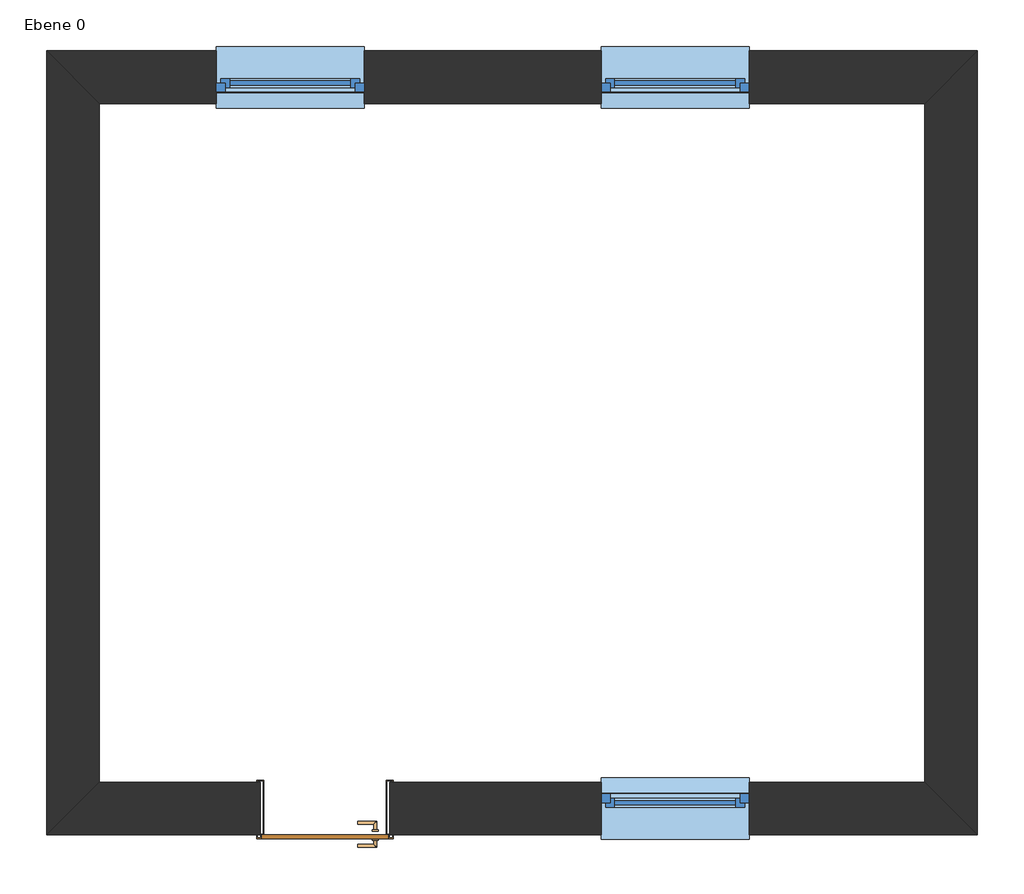
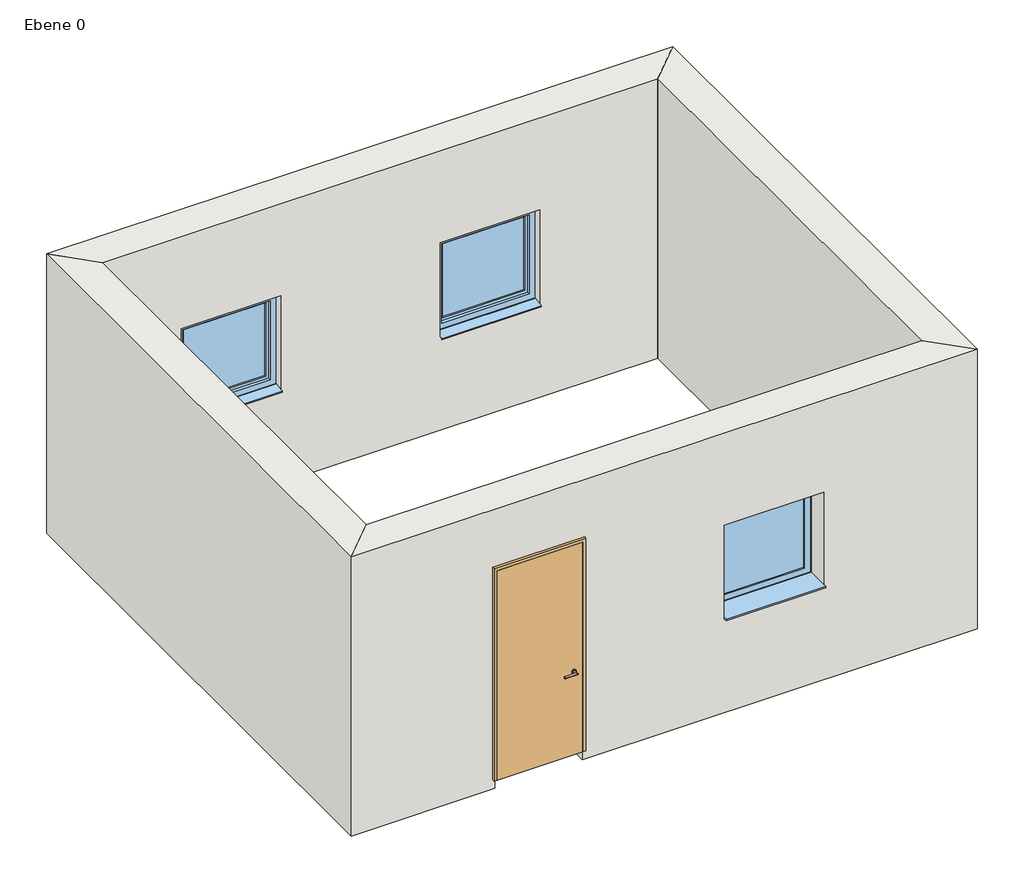
# One storey: 4 walls, 3 windows, 1 door.
"""IFC4 building model written with IfcOpenShell, lengths in millimetres."""

import ifcopenshell
import ifcopenshell.guid

model = None  # the IFC model being written
_history = None  # IfcOwnerHistory: only IFC2X3 demands one
_inside = {}  # id of a spatial element -> (the spatial element, [elements in it])
_under = {}  # id of a project, library or spatial element -> (it, [spatial elements below it])
_declared = {}  # id of a project -> (the project, [libraries it declares])
_typed = {}  # id of a type object -> (the type object, [elements of that type])
_made_of = {}  # id of a material, layer set ... -> (it, [elements and type objects made of it])


def new_model(schema):
    """Start an empty IFC model of exactly this schema.

    Asked for "IFC4X3", IfcOpenShell would pick the latest addendum, in which some entities
    have other attributes; the version numbers below select the first issue.
    IFC2X3 requires an IfcOwnerHistory on every rooted entity: one is made here for all.
    """
    global model, _history
    if schema == "IFC4X3":
        model = ifcopenshell.file(schema_version=(4, 3, 0, 0))
    else:
        model = ifcopenshell.file(schema=schema)
    _inside.clear()
    _under.clear()
    _declared.clear()
    _typed.clear()
    _made_of.clear()
    _history = None
    if model.schema == "IFC2X3":
        org = make("IfcOrganization", Name="unknown")
        user = make(
            "IfcPersonAndOrganization",
            ThePerson=make("IfcPerson", FamilyName="unknown"),
            TheOrganization=org,
        )
        app = make(
            "IfcApplication",
            ApplicationDeveloper=org,
            Version="unknown",
            ApplicationFullName="unknown",
            ApplicationIdentifier="unknown",
        )
        _history = make(
            "IfcOwnerHistory",
            OwningUser=user,
            OwningApplication=app,
            ChangeAction="ADDED",
            CreationDate=0,
        )
    return model


def make(cls, **values):
    """One entity of the class cls with the attributes given. An attribute that is None is left unset."""
    return model.create_entity(
        cls, **{name: value for name, value in values.items() if value is not None}
    )


def rooted(cls, **values):
    """An entity with a GlobalId (a new one), such as an element, a storey or a relation."""
    return make(cls, GlobalId=ifcopenshell.guid.new(), OwnerHistory=_history, **values)


def si_unit(unit_type, name, prefix=None):
    """IfcSIUnit, for example si_unit("LENGTHUNIT", "METRE", prefix="MILLI")."""
    return make("IfcSIUnit", UnitType=unit_type, Prefix=prefix, Name=name)


def assignment(units):
    """IfcUnitAssignment: the units of a project."""
    return None if units is None else make("IfcUnitAssignment", Units=units)


def point(xyz):
    """IfcCartesianPoint."""
    return None if xyz is None else make("IfcCartesianPoint", Coordinates=xyz)


def direction(xyz):
    """IfcDirection."""
    return None if xyz is None else make("IfcDirection", DirectionRatios=xyz)


def frame(location, z_axis=None, x_axis=None):
    """IfcAxis2Placement3D, a coordinate frame: its origin and axes. An axis left out is left unset."""
    return make(
        "IfcAxis2Placement3D",
        Location=point(location),
        Axis=direction(z_axis),
        RefDirection=direction(x_axis),
    )


def frame_2d(location, x_axis=None):
    """IfcAxis2Placement2D, a coordinate frame in the plane: its origin and x axis."""
    return make(
        "IfcAxis2Placement2D", Location=point(location), RefDirection=direction(x_axis)
    )


def origin():
    """The frame at (0, 0, 0) with its axes left unset."""
    return frame((0.0, 0.0, 0.0))


def origin_with_axes():
    """The frame at (0, 0, 0) with the z axis (0, 0, 1) and the x axis (1, 0, 0) written out."""
    return frame((0.0, 0.0, 0.0), z_axis=(0.0, 0.0, 1.0), x_axis=(1.0, 0.0, 0.0))


def place(relative_to, where):
    """IfcLocalPlacement: puts the frame where relative to a parent placement (None: the world)."""
    return make(
        "IfcLocalPlacement", PlacementRelTo=relative_to, RelativePlacement=where
    )


def context(
    kind, dimensions, precision=None, world=None, true_north=None, identifier=None
):
    """IfcGeometricRepresentationContext, for example the 3D "Model" context."""
    return make(
        "IfcGeometricRepresentationContext",
        ContextIdentifier=identifier,
        ContextType=kind,
        CoordinateSpaceDimension=dimensions,
        Precision=precision,
        WorldCoordinateSystem=world,
        TrueNorth=true_north,
    )


def project(units=None, contexts=None):
    """IfcProject with its units and contexts."""
    return rooted(
        "IfcProject",
        Name="project",
        RepresentationContexts=contexts,
        UnitsInContext=assignment(units),
    )


def spatial(cls, under=None, at=None, **own):
    """A site, building, storey or space (cls), placed at a placement, below another one or the project."""
    s = rooted(cls, ObjectPlacement=at, **own)
    if under is not None:
        _under.setdefault(under.id(), (under, []))[1].append(s)
    return s


def polyline(points):
    """IfcPolyline through the points."""
    return make("IfcPolyline", Points=[point(p) for p in points])


def circle_curve(where, radius):
    """IfcCircle in the frame where."""
    return make("IfcCircle", Position=where, Radius=radius)


def ellipse_curve(where, semi_axis1, semi_axis2):
    """IfcEllipse in the frame where."""
    return make(
        "IfcEllipse", Position=where, SemiAxis1=semi_axis1, SemiAxis2=semi_axis2
    )


def trimmed(basis, trim1, trim2, sense, master):
    """IfcTrimmedCurve: the piece of a basis curve between two trims."""
    return make(
        "IfcTrimmedCurve",
        BasisCurve=basis,
        Trim1=trim1,
        Trim2=trim2,
        SenseAgreement=sense,
        MasterRepresentation=master,
    )


def segment(curve, same_sense, transition):
    """IfcCompositeCurveSegment."""
    return make(
        "IfcCompositeCurveSegment",
        Transition=transition,
        SameSense=same_sense,
        ParentCurve=curve,
    )


def composite_curve(segments, self_intersect=None):
    """IfcCompositeCurve: segments joined end to end."""
    return make("IfcCompositeCurve", Segments=segments, SelfIntersect=self_intersect)


def outline(outer, holes=None, kind="AREA"):
    """IfcArbitraryClosedProfileDef: a profile drawn as a closed curve; with holes, ...WithVoids."""
    if holes is None:
        return make("IfcArbitraryClosedProfileDef", ProfileType=kind, OuterCurve=outer)
    return make(
        "IfcArbitraryProfileDefWithVoids",
        ProfileType=kind,
        OuterCurve=outer,
        InnerCurves=holes,
    )


def extrude(swept, where, along, depth):
    """IfcExtrudedAreaSolid: the profile swept, set in the frame where, extruded along a direction by depth."""
    return make(
        "IfcExtrudedAreaSolid",
        SweptArea=swept,
        Position=where,
        ExtrudedDirection=direction(along),
        Depth=depth,
    )


def faces_of(points, faces, orient=None, outer=None):
    """IfcFace entities. A face is a list of loops; a loop is a list of indices into points, from 0.

    orient and outer hold one flag for each loop. By default every Orientation is true, the
    first loop of a face is its IfcFaceOuterBound and the others are IfcFaceBound.
    """
    made = []
    for i, loops in enumerate(faces):
        bounds = []
        for j, loop in enumerate(loops):
            is_outer = j == 0 if outer is None else outer[i][j]
            bounds.append(
                make(
                    "IfcFaceOuterBound" if is_outer else "IfcFaceBound",
                    Bound=make("IfcPolyLoop", Polygon=[points[k] for k in loop]),
                    Orientation=True if orient is None else orient[i][j],
                )
            )
        made.append(make("IfcFace", Bounds=bounds))
    return made


def faceted_brep(points, faces, orient=None, outer=None, voids=None):
    """IfcFacetedBrep: a solid bounded by flat faces; with voids (closed shells), ...WithVoids."""
    shared = [point(p) for p in points]
    hull = make("IfcClosedShell", CfsFaces=faces_of(shared, faces, orient, outer))
    if voids is None:
        return make("IfcFacetedBrep", Outer=hull)
    return make(
        "IfcFacetedBrepWithVoids",
        Outer=hull,
        Voids=[
            make(cls, CfsFaces=faces_of(shared, fs, o, b)) for cls, fs, o, b in voids
        ],
    )


def shape(context_of_items, identifier, shape_type, items):
    """IfcShapeRepresentation: the items that make up one representation, for example the "Body"."""
    return make(
        "IfcShapeRepresentation",
        ContextOfItems=context_of_items,
        RepresentationIdentifier=identifier,
        RepresentationType=shape_type,
        Items=items,
    )


def source(mapping_origin, context_of_items, identifier, shape_type, items):
    """IfcRepresentationMap: a shape defined once, which mapped items show again and again."""
    return make(
        "IfcRepresentationMap",
        MappingOrigin=mapping_origin,
        MappedRepresentation=shape(context_of_items, identifier, shape_type, items),
    )


def transform(
    local_origin,
    x_axis=None,
    y_axis=None,
    z_axis=None,
    scale=None,
    scale2=None,
    scale3=None,
    uniform=True,
):
    """IfcCartesianTransformationOperator3D, or its non-uniform kind. x_axis, y_axis, z_axis: its Axis1, 2, 3."""
    if uniform:
        return make(
            "IfcCartesianTransformationOperator3D",
            Axis1=direction(x_axis),
            Axis2=direction(y_axis),
            LocalOrigin=point(local_origin),
            Scale=scale,
            Axis3=direction(z_axis),
        )
    return make(
        "IfcCartesianTransformationOperator3DnonUniform",
        Axis1=direction(x_axis),
        Axis2=direction(y_axis),
        LocalOrigin=point(local_origin),
        Scale=scale,
        Axis3=direction(z_axis),
        Scale2=scale2,
        Scale3=scale3,
    )


def mapped(mapping_source, mapping_target):
    """IfcMappedItem: shows the shape of a source again, moved by a transform."""
    return make(
        "IfcMappedItem", MappingSource=mapping_source, MappingTarget=mapping_target
    )


def made_of(thing, what):
    """Note that an element or type object is made of a material, layer set ...; save() writes the relation."""
    if what is not None:
        _made_of.setdefault(what.id(), (what, []))[1].append(thing)
    return thing


def element(
    cls,
    number,
    at=None,
    inside=None,
    cuts=None,
    type_object=None,
    material=None,
    context=None,
    identifier="Body",
    shape_type=None,
    held_by="IfcProductDefinitionShape",
    body=None,
    shapes=None,
    **own,
):
    """One element of the class cls, such as IfcWall. Its Tag is "e" and its number.

    at: its placement. inside: the storey or other place that contains it. cuts: it is an
    opening in that element (IfcRelVoidsElement). A single representation is given by context,
    identifier, shape_type and body (its items); several are given by shapes. held_by: the class
    of the entity that holds the representations. save() writes the other relations.
    """
    e = rooted(cls, Tag="e%d" % number, ObjectPlacement=at, **own)
    if body is not None:
        shapes = [shape(context, identifier, shape_type, body)]
    if shapes is not None:
        e.Representation = make(held_by, Representations=shapes)
    if inside is not None:
        _inside.setdefault(inside.id(), (inside, []))[1].append(e)
    if cuts is not None:
        rooted(
            "IfcRelVoidsElement", RelatingBuildingElement=cuts, RelatedOpeningElement=e
        )
    if type_object is not None:
        _typed.setdefault(type_object.id(), (type_object, []))[1].append(e)
    return made_of(e, material)


def aggregate(whole, parts):
    """IfcRelAggregates: a whole, such as a stair, and the parts it consists of."""
    return rooted("IfcRelAggregates", RelatingObject=whole, RelatedObjects=parts)


def save(model, path):
    """Write the relations noted so far, then the file.

    IfcRelAggregates (storeys below a building ...), IfcRelContainedInSpatialStructure (elements
    in a storey), IfcRelDefinesByType, IfcRelAssociatesMaterial and IfcRelDeclares: one each for
    every whole, place, type object, material and project.
    """
    for whole, parts in _under.values():
        aggregate(whole, parts)
    for where, things in _inside.values():
        rooted(
            "IfcRelContainedInSpatialStructure",
            RelatedElements=things,
            RelatingStructure=where,
        )
    for kind, things in _typed.values():
        rooted("IfcRelDefinesByType", RelatedObjects=things, RelatingType=kind)
    for what, things in _made_of.values():
        rooted("IfcRelAssociatesMaterial", RelatedObjects=things, RelatingMaterial=what)
    for by, libraries in _declared.values():
        rooted("IfcRelDeclares", RelatingContext=by, RelatedDefinitions=libraries)
    model.write(path)


def plane_surface(at):
    """IfcPlane: the flat surface through the origin of the frame at, square to its z axis."""
    return make("IfcPlane", Position=at)


def cylinder_surface(at, radius):
    """IfcCylindricalSurface: all points at the distance radius from the z axis of the frame at."""
    return make("IfcCylindricalSurface", Position=at, Radius=radius)


def advanced_brep(points, edges, surfaces, faces):
    """IfcAdvancedBrep: a solid bounded by faces that lie on surfaces and meet in shared edges.

    An edge is (start, end): straight between two places in points (the first is 0);
    or (start, end, curve); or (start, end, curve, False) where it runs against its curve.
    A face is (place in surfaces, loops), or (place, loops, False) where it looks against
    its surface's normal. A loop lists edges by number (the first is 1), with a minus sign
    where the edge is run from its end to its start. The first loop is the outer one.
    """
    corners = [point(p) for p in points]
    vertices = [make("IfcVertexPoint", VertexGeometry=c) for c in corners]
    made = []
    for start, end, *more in edges:
        made.append(
            make(
                "IfcEdgeCurve",
                EdgeStart=vertices[start],
                EdgeEnd=vertices[end],
                EdgeGeometry=more[0] if more else make("IfcPolyline", Points=[corners[start], corners[end]]),
                SameSense=more[1] if len(more) > 1 else True,
            )
        )
    hull = []
    for where, loops, *sense in faces:
        bounds = []
        for j, loop in enumerate(loops):
            ring = [make("IfcOrientedEdge", EdgeElement=made[abs(k) - 1], Orientation=k > 0) for k in loop]
            bounds.append(
                make(
                    "IfcFaceOuterBound" if j == 0 else "IfcFaceBound",
                    Bound=make("IfcEdgeLoop", EdgeList=ring),
                    Orientation=True,
                )
            )
        hull.append(make("IfcAdvancedFace", Bounds=bounds, FaceSurface=surfaces[where], SameSense=sense[0] if sense else True))
    return make("IfcAdvancedBrep", Outer=make("IfcClosedShell", CfsFaces=hull))


def door_88_5_x_2_26_80f06d6c(model_context):
    return source(origin(), model_context, "Body", "SolidModel", [
        advanced_brep(
        [(-352.5, 169.4346141, 1000.0), (-332.5, 169.4346141, 1000.0), (-352.5, 99.4346141, 1000.0), (-332.5, 119.4346141, 1000.0), (-222.5, 99.4346141, 1000.0), (-222.5, 119.4346141, 1000.0)],
        [
            (0, 1, circle_curve(frame((-342.5, 169.4346141, 1000.0), z_axis=(0.0, 1.0, 0.0), x_axis=(1.0, 0.0, 0.0)), 10.0)),
            (1, 0, circle_curve(frame((-342.5, 169.4346141, 1000.0), z_axis=(0.0, 1.0, 0.0), x_axis=(1.0, 0.0, 0.0)), 10.0)),
            (0, 2),
            (2, 3, ellipse_curve(frame((-342.5, 109.4346141, 1000.0), z_axis=(-0.7071067811865385, 0.7071067811865565, 0.0), x_axis=(0.7071067811865563, 0.7071067811865386, 0.0)), 14.1421356, 10.0)),
            (3, 1),
            (3, 2, ellipse_curve(frame((-342.5, 109.4346141, 1000.0), z_axis=(-0.7071067811865385, 0.7071067811865565, 0.0), x_axis=(0.7071067811865563, 0.7071067811865386, 0.0)), 14.1421356, 10.0)),
            (4, 5, circle_curve(frame((-222.5, 109.4346141, 1000.0), z_axis=(1.0, 0.0, 0.0), x_axis=(0.0, 1.0, 0.0)), 10.0)),
            (5, 4, circle_curve(frame((-222.5, 109.4346141, 1000.0), z_axis=(1.0, 0.0, 0.0), x_axis=(0.0, 1.0, 0.0)), 10.0)),
            (2, 4),
            (5, 3),
        ],
        [
            plane_surface(frame((-342.5, 169.4346141, -287.7526403), z_axis=(0.0, 1.0, 0.0), x_axis=(0.0, 0.0, 1.0))),
            cylinder_surface(frame((-342.5, 169.4346141, 1000.0), z_axis=(0.0, 1.0, 0.0), x_axis=(1.0, 0.0, 0.0)), 10.0),
            plane_surface(frame((-222.5, 109.4346141, -287.7526403), z_axis=(1.0, 0.0, 0.0), x_axis=(0.0, 0.0, 1.0))),
            cylinder_surface(frame((-342.5, 109.4346141, 1000.0), z_axis=(-1.0, 0.0, 0.0), x_axis=(0.0, 1.0, 0.0)), 10.0),
        ],
        [
            (0, [[1, 2]]),
            (1, [[-1, 3, 4, 5]]),
            (1, [[-2, -5, 6, -3]]),
            (2, [[7, 8]]),
            (3, [[-4, 9, -8, 10]]),
            (3, [[-6, -10, -7, -9]]),
        ],
    ),
        advanced_brep(
        [(-332.5, 229.4346141, 1000.0), (-352.5, 229.4346141, 1000.0), (-332.5, 259.4346141, 1000.0), (-352.5, 279.4346141, 1000.0), (-222.5, 259.4346141, 1000.0), (-222.5, 279.4346141, 1000.0)],
        [
            (0, 1, circle_curve(frame((-342.5, 229.4346141, 1000.0), z_axis=(0.0, -1.0, 0.0), x_axis=(-1.0, 0.0, 0.0)), 10.0)),
            (1, 0, circle_curve(frame((-342.5, 229.4346141, 1000.0), z_axis=(0.0, -1.0, 0.0), x_axis=(-1.0, 0.0, 0.0)), 10.0)),
            (0, 2),
            (2, 3, ellipse_curve(frame((-342.5, 269.4346141, 1000.0), z_axis=(-0.7071067811865475, -0.7071067811865475, 0.0), x_axis=(0.7071067811865474, -0.7071067811865476, 0.0)), 14.1421356, 10.0)),
            (3, 1),
            (3, 2, ellipse_curve(frame((-342.5, 269.4346141, 1000.0), z_axis=(-0.7071067811865475, -0.7071067811865475, 0.0), x_axis=(0.7071067811865474, -0.7071067811865476, 0.0)), 14.1421356, 10.0)),
            (4, 5, circle_curve(frame((-222.5, 269.4346141, 1000.0), z_axis=(1.0, 0.0, 0.0), x_axis=(0.0, 1.0, 0.0)), 10.0)),
            (5, 4, circle_curve(frame((-222.5, 269.4346141, 1000.0), z_axis=(1.0, 0.0, 0.0), x_axis=(0.0, 1.0, 0.0)), 10.0)),
            (2, 4),
            (5, 3),
        ],
        [
            plane_surface(frame((-342.5, 229.4346141, -287.7526403), z_axis=(0.0, -1.0, 0.0), x_axis=(0.0, 0.0, 1.0))),
            cylinder_surface(frame((-342.5, 229.4346141, 1000.0), z_axis=(0.0, -1.0, 0.0), x_axis=(-1.0, 0.0, 0.0)), 10.0),
            plane_surface(frame((-222.5, 269.4346141, -287.7526403), z_axis=(1.0, 0.0, 0.0), x_axis=(0.0, 0.0, 1.0))),
            cylinder_surface(frame((-342.5, 269.4346141, 1000.0), z_axis=(-1.0, 0.0, 0.0), x_axis=(0.0, 1.0, 0.0)), 10.0),
        ],
        [
            (0, [[1, 2]]),
            (1, [[-1, 3, 4, 5]]),
            (1, [[-2, -5, 6, -3]]),
            (2, [[7, 8]]),
            (3, [[-4, 9, -8, 10]]),
            (3, [[-6, -10, -7, -9]]),
        ],
    ),
        extrude(outline(composite_curve([segment(trimmed(circle_curve(frame_2d((1000.0, -342.5)), 20.0), [point((1000.0, -362.5))], [point((1000.0, -322.5))], False, "CARTESIAN"), True, "CONTINUOUS"), segment(trimmed(circle_curve(frame_2d((1000.0, -342.5)), 20.0), [point((1000.0, -322.5))], [point((1000.0, -362.5))], False, "CARTESIAN"), True, "CONTINUOUS")], self_intersect=False)), frame((0.0, 159.4346141, 0.0), z_axis=(0.0, 1.0, 0.0), x_axis=(0.0, 0.0, 1.0)), (0.0, 0.0, 1.0), 10.0),
        extrude(outline(composite_curve([segment(trimmed(circle_curve(frame_2d((1000.0, -342.5)), 20.0), [point((1000.0, -362.5))], [point((1000.0, -322.5))], False, "CARTESIAN"), True, "CONTINUOUS"), segment(trimmed(circle_curve(frame_2d((1000.0, -342.5)), 20.0), [point((1000.0, -322.5))], [point((1000.0, -362.5))], False, "CARTESIAN"), True, "CONTINUOUS")], self_intersect=False)), frame((0.0, 219.4346141, 0.0), z_axis=(0.0, 1.0, 0.0), x_axis=(0.0, 0.0, 1.0)), (0.0, 0.0, 1.0), 10.0),
        extrude(outline(polyline([(432.5, 194.4346141), (-432.5, 194.4346141), (-432.5, 219.4346141), (432.5, 219.4346141), (432.5, 194.4346141)])), frame((0.0, 0.0, 100.0), z_axis=(0.0, 0.0, 1.0), x_axis=(1.0, 0.0, 0.0)), (0.0, 0.0, 1.0), 2250.0),
        faceted_brep([(466.9603207, -180.5653859, 100.0), (417.5, -180.5653859, 100.0), (417.5, 194.4346141, 100.0), (432.5, 194.4346141, 100.0), (432.5, 219.4346141, 100.0), (466.9603207, 219.4346141, 100.0), (466.9603207, 194.4346141, 100.0), (461.9603207, 194.4346141, 100.0), (461.9603207, 214.4346141, 100.0), (437.5, 214.4346141, 100.0), (437.5, 189.4346141, 100.0), (422.5, 189.4346141, 100.0), (422.5, -175.5653859, 100.0), (461.9603207, -175.5653859, 100.0), (461.9603207, -165.5653859, 100.0), (466.9603207, -165.5653859, 100.0), (466.9603207, -180.5653859, 2384.4603207), (-466.9603207, -180.5653859, 2384.4603207), (-466.9603207, -180.5653859, 100.0), (-417.5, -180.5653859, 100.0), (-417.5, -180.5653859, 2335.0), (417.5, -180.5653859, 2335.0), (417.5, 194.4346141, 2335.0), (-417.5, 194.4346141, 2335.0), (-417.5, 194.4346141, 100.0), (-432.5, 194.4346141, 100.0), (-432.5, 194.4346141, 2350.0), (432.5, 194.4346141, 2350.0), (432.5, 219.4346141, 2350.0), (-432.5, 219.4346141, 2350.0), (-432.5, 219.4346141, 100.0), (-466.9603207, 219.4346141, 100.0), (-466.9603207, 219.4346141, 2384.4603207), (466.9603207, 219.4346141, 2384.4603207), (466.9603207, 194.4346141, 2384.4603207), (-466.9603207, 194.4346141, 2384.4603207), (-466.9603207, 194.4346141, 100.0), (-461.9603207, 194.4346141, 100.0), (-461.9603207, 194.4346141, 2379.4603207), (461.9603207, 194.4346141, 2379.4603207), (461.9603207, 214.4346141, 2379.4603207), (-461.9603207, 214.4346141, 2379.4603207), (-461.9603207, 214.4346141, 100.0), (-437.5, 214.4346141, 100.0), (-437.5, 214.4346141, 2355.0), (437.5, 214.4346141, 2355.0), (437.5, 189.4346141, 2355.0), (-437.5, 189.4346141, 2355.0), (-437.5, 189.4346141, 100.0), (-422.5, 189.4346141, 100.0), (-422.5, 189.4346141, 2340.0), (422.5, 189.4346141, 2340.0), (422.5, -175.5653859, 2340.0), (-422.5, -175.5653859, 2340.0), (-422.5, -175.5653859, 100.0), (-461.9603207, -175.5653859, 100.0), (-461.9603207, -175.5653859, 2379.4603207), (461.9603207, -175.5653859, 2379.4603207), (461.9603207, -165.5653859, 2379.4603207), (-461.9603207, -165.5653859, 2379.4603207), (-461.9603207, -165.5653859, 100.0), (-466.9603207, -165.5653859, 100.0), (-466.9603207, -165.5653859, 2384.4603207), (466.9603207, -165.5653859, 2384.4603207)], [[[0, 1, 2, 3, 4, 5, 6, 7, 8, 9, 10, 11, 12, 13, 14, 15]], [[1, 0, 16, 17, 18, 19, 20, 21]], [[2, 1, 21, 22]], [[3, 2, 22, 23, 24, 25, 26, 27]], [[4, 3, 27, 28]], [[5, 4, 28, 29, 30, 31, 32, 33]], [[6, 5, 33, 34]], [[7, 6, 34, 35, 36, 37, 38, 39]], [[8, 7, 39, 40]], [[9, 8, 40, 41, 42, 43, 44, 45]], [[10, 9, 45, 46]], [[11, 10, 46, 47, 48, 49, 50, 51]], [[12, 11, 51, 52]], [[13, 12, 52, 53, 54, 55, 56, 57]], [[14, 13, 57, 58]], [[15, 14, 58, 59, 60, 61, 62, 63]], [[0, 15, 63, 16]], [[17, 62, 61, 18]], [[18, 61, 60, 55, 54, 49, 48, 43, 42, 37, 36, 31, 30, 25, 24, 19]], [[23, 20, 19, 24]], [[29, 26, 25, 30]], [[35, 32, 31, 36]], [[41, 38, 37, 42]], [[47, 44, 43, 48]], [[53, 50, 49, 54]], [[59, 56, 55, 60]], [[22, 21, 20, 23]], [[28, 27, 26, 29]], [[34, 33, 32, 35]], [[40, 39, 38, 41]], [[46, 45, 44, 47]], [[52, 51, 50, 53]], [[58, 57, 56, 59]], [[16, 63, 62, 17]]]),
    ])


def fenster_1_flg_variabel_fenster_1_flg_variabel_3_8a378bad(model_context):
    return source(origin(), model_context, "Body", "SolidModel", [
        extrude(outline(polyline([(2010.0, 505.0), (2010.0, -505.0), (1000.0, -505.0), (1000.0, 505.0), (2010.0, 505.0)]), holes=[polyline([(1930.0, 445.0), (1080.0, 445.0), (1080.0, -445.0), (1930.0, -445.0), (1930.0, 445.0)])]), frame((0.0, 40.0, 0.0), z_axis=(0.0, 1.0, 0.0), x_axis=(0.0, 0.0, 1.0)), (0.0, 0.0, 1.0), 60.0),
        faceted_brep([(475.0, 40.0, 1960.0), (475.0, 10.0, 1960.0), (475.0, 10.0, 1050.0), (475.0, 40.0, 1050.0), (-475.0, 10.0, 1960.0), (-475.0, 10.0, 1050.0), (415.0, 10.0, 1110.0), (-415.0, 10.0, 1110.0), (-415.0, 10.0, 1900.0), (415.0, 10.0, 1900.0), (-475.0, 40.0, 1050.0), (-475.0, 40.0, 1960.0), (445.0, 40.0, 1930.0), (-445.0, 40.0, 1930.0), (-445.0, 40.0, 1080.0), (445.0, 40.0, 1080.0), (445.0, 70.0, 1930.0), (445.0, 70.0, 1080.0), (-445.0, 70.0, 1080.0), (-445.0, 70.0, 1930.0), (415.0, 70.0, 1900.0), (-415.0, 70.0, 1900.0), (-415.0, 70.0, 1110.0), (415.0, 70.0, 1110.0)], [[[0, 1, 2, 3]], [[1, 4, 5, 2], [6, 7, 8, 9]], [[3, 2, 5, 10]], [[3, 10, 11, 0], [12, 13, 14, 15]], [[16, 12, 15, 17]], [[17, 15, 14, 18]], [[17, 18, 19, 16], [20, 21, 22, 23]], [[9, 20, 23, 6]], [[6, 23, 22, 7]], [[10, 5, 4, 11]], [[18, 14, 13, 19]], [[7, 22, 21, 8]], [[11, 4, 1, 0]], [[19, 13, 12, 16]], [[8, 21, 20, 9]]]),
        extrude(outline(polyline([(-505.0, -210.0), (-505.0, 40.0), (505.0, 40.0), (505.0, -210.0), (-505.0, -210.0)])), frame((0.0, 0.0, 1005.0), z_axis=(0.0, 0.0, 1.0), x_axis=(1.0, 0.0, 0.0)), (0.0, 0.0, 1.0), 15.0),
        extrude(outline(polyline([(110.0221543, 1020.0), (210.0, 1000.0), (210.0, 990.0), (208.0, 990.0), (208.0, 998.3604634), (109.8240723, 1018.0), (100.0, 1018.0), (100.0, 1020.0), (110.0221543, 1020.0)])), frame((-505.0, 0.0, 0.0), z_axis=(1.0, 0.0, 0.0), x_axis=(0.0, 1.0, 0.0)), (0.0, 0.0, 1.0), 1010.0),
        extrude(outline(polyline([(415.0, 25.0), (-415.0, 25.0), (-415.0, 55.0), (415.0, 55.0), (415.0, 25.0)])), frame((0.0, 0.0, 1110.0), z_axis=(0.0, 0.0, 1.0), x_axis=(1.0, 0.0, 0.0)), (0.0, 0.0, 1.0), 790.0),
    ])


model = new_model("IFC4")

# Units and contexts
model_context = context("Model", 3, world=origin())
ifc_project = project(units=[si_unit("LENGTHUNIT", "METRE", prefix="MILLI")], contexts=[model_context])

# Site, building, storey
site = spatial("IfcSite", under=ifc_project)
building = spatial("IfcBuilding", under=site)
storey = spatial("IfcBuildingStorey", under=building, Name="Ebene 0", Elevation=0.0)

# Door
placement = place(None, origin())
door_88_5_x_2_26_shape = door_88_5_x_2_26_80f06d6c(model_context)
element("IfcDoor", 1, ObjectType="Drehflügel 1-flg - Stahlzarge : 88.5 x 2.26", at=placement, inside=storey, context=model_context, shape_type="MappedRepresentation", body=[
    mapped(door_88_5_x_2_26_shape, transform((-2223.9979049, -761.1961342, 0.0), x_axis=(-1.0, 0.0, 0.0), y_axis=(0.0, -1.0, 0.0), z_axis=(0.0, 0.0, 1.0))),
])

# Walls
element("IfcWall", 2, ObjectType="MW 24.0 WD 12.0", at=placement, inside=storey, context=model_context, shape_type="Brep", body=[
    faceted_brep([(-3766.4979049, 4044.3692517, 0.0), (1873.5020951, 4044.3692517, 0.0), (1873.5020951, 4044.3692517, 3000.0), (-3766.4979049, 4044.3692517, 3000.0), (673.5020951, 4044.3692517, 1000.0), (-336.4979049, 4044.3692517, 1000.0), (-336.4979049, 4044.3692517, 2010.0), (673.5020951, 4044.3692517, 2010.0), (-1956.4979049, 4044.3692517, 1000.0), (-2966.4979049, 4044.3692517, 1000.0), (-2966.4979049, 4044.3692517, 2010.0), (-1956.4979049, 4044.3692517, 2010.0), (-4126.4979049, 4404.3692517, 0.0), (-4126.4979049, 4404.3692517, 3000.0), (2233.5020951, 4404.3692517, 3000.0), (2233.5020951, 4404.3692517, 0.0), (673.5020951, 4404.3692517, 1000.0), (673.5020951, 4404.3692517, 2010.0), (-336.4979049, 4404.3692517, 2010.0), (-336.4979049, 4404.3692517, 1000.0), (-1956.4979049, 4404.3692517, 1000.0), (-1956.4979049, 4404.3692517, 2010.0), (-2966.4979049, 4404.3692517, 2010.0), (-2966.4979049, 4404.3692517, 1000.0)], [[[0, 1, 2, 3], [4, 5, 6, 7], [8, 9, 10, 11]], [[12, 13, 14, 15], [16, 17, 18, 19], [20, 21, 22, 23]], [[1, 0, 12, 15]], [[3, 2, 14, 13]], [[17, 16, 4, 7]], [[18, 17, 7, 6]], [[19, 18, 6, 5]], [[16, 19, 5, 4]], [[21, 20, 8, 11]], [[22, 21, 11, 10]], [[23, 22, 10, 9]], [[20, 23, 9, 8]], [[0, 3, 13, 12]], [[2, 1, 15, 14]]]),
])
element("IfcWall", 3, ObjectType="MW 24.0 WD 12.0", at=placement, inside=storey, context=model_context, shape_type="SweptSolid", body=[
    extrude(outline(polyline([(1873.5020951, -595.6307483), (1873.5020951, 4044.3692517), (2233.5020951, 4404.3692517), (2233.5020951, -955.6307483), (1873.5020951, -595.6307483)])), origin_with_axes(), (0.0, 0.0, 1.0), 3000.0),
])
element("IfcWall", 4, ObjectType="MW 24.0 WD 12.0", at=placement, inside=storey, context=model_context, shape_type="Brep", body=[
    faceted_brep([(-3766.4979049, -595.6307483, 3000.0), (1873.5020951, -595.6307483, 3000.0), (1873.5020951, -595.6307483, 0.0), (-1781.4979049, -595.6307483, 0.0), (-1781.4979049, -595.6307483, 2360.0), (-2666.4979049, -595.6307483, 2360.0), (-2666.4979049, -595.6307483, 0.0), (-3766.4979049, -595.6307483, 0.0), (-336.4979049, -595.6307483, 1000.0), (673.5020951, -595.6307483, 1000.0), (673.5020951, -595.6307483, 2010.0), (-336.4979049, -595.6307483, 2010.0), (2233.5020951, -955.6307483, 3000.0), (-4126.4979049, -955.6307483, 3000.0), (-4126.4979049, -955.6307483, 0.0), (-2666.4979049, -955.6307483, 0.0), (-2666.4979049, -955.6307483, 2360.0), (-1781.4979049, -955.6307483, 2360.0), (-1781.4979049, -955.6307483, 0.0), (2233.5020951, -955.6307483, 0.0), (-336.4979049, -955.6307483, 1000.0), (-336.4979049, -955.6307483, 2010.0), (673.5020951, -955.6307483, 2010.0), (673.5020951, -955.6307483, 1000.0)], [[[0, 1, 2, 3, 4, 5, 6, 7], [8, 9, 10, 11]], [[12, 13, 14, 15, 16, 17, 18, 19], [20, 21, 22, 23]], [[2, 19, 18, 3]], [[14, 7, 6, 15]], [[1, 0, 13, 12]], [[5, 16, 15, 6]], [[16, 5, 4, 17]], [[17, 4, 3, 18]], [[21, 20, 8, 11]], [[22, 21, 11, 10]], [[23, 22, 10, 9]], [[20, 23, 9, 8]], [[2, 1, 12, 19]], [[0, 7, 14, 13]]]),
])
element("IfcWall", 5, ObjectType="MW 24.0 WD 12.0", at=placement, inside=storey, context=model_context, shape_type="SweptSolid", body=[
    extrude(outline(polyline([(-3766.4979049, 4044.3692517), (-3766.4979049, -595.6307483), (-4126.4979049, -955.6307483), (-4126.4979049, 4404.3692517), (-3766.4979049, 4044.3692517)])), origin_with_axes(), (0.0, 0.0, 1.0), 3000.0),
])

# Windows
fenster_1_flg_variabel_fenster_1_flg_variabel_3_shape = fenster_1_flg_variabel_fenster_1_flg_variabel_3_8a378bad(model_context)
element("IfcWindow", 6, ObjectType="Fenster 1-flg - Variabel : Fenster 1-flg - Variabel 3", at=placement, inside=storey, context=model_context, shape_type="MappedRepresentation", body=[
    mapped(fenster_1_flg_variabel_fenster_1_flg_variabel_3_shape, transform((168.5020951, -775.6307483, 0.0), x_axis=(1.0, 0.0, 0.0), y_axis=(0.0, 1.0, 0.0), z_axis=(0.0, 0.0, 1.0))),
])
element("IfcWindow", 7, ObjectType="Fenster 1-flg - Variabel : Fenster 1-flg - Variabel 3", at=placement, inside=storey, context=model_context, shape_type="MappedRepresentation", body=[
    mapped(fenster_1_flg_variabel_fenster_1_flg_variabel_3_shape, transform((168.5020951, 4224.3692517, 0.0), x_axis=(-1.0, 0.0, 0.0), y_axis=(0.0, -1.0, 0.0), z_axis=(0.0, 0.0, 1.0))),
])
element("IfcWindow", 8, ObjectType="Fenster 1-flg - Variabel : Fenster 1-flg - Variabel 3", at=placement, inside=storey, context=model_context, shape_type="MappedRepresentation", body=[
    mapped(fenster_1_flg_variabel_fenster_1_flg_variabel_3_shape, transform((-2461.4979049, 4224.3692517, 0.0), x_axis=(-1.0, 0.0, 0.0), y_axis=(0.0, -1.0, 0.0), z_axis=(0.0, 0.0, 1.0))),
])

save(model, "model.ifc")

# Revit data of these elements
# Project information
#   Testproperty = "TestpropertyValue"
#   Projektausgabedatum = "Projekt Datum"
#   Projektstatus = "Projektstatus"
#   Auftraggeber = "Walter Beispiel"
#   Projektadresse = "Zufallweg 2"
#   Projektname = "Projektname"
#   Projektnummer = "Projektnummer"
#   Verfasser Firma 1 = "Firma 1"
#   Verfasser Firma 2 = "Firma 2"
#   Verfasser PLZ Ort = "PLZ Ort"
#   Verfasser Strasse = "Strasse"
#   Verfasser Telefon = "Telefon"
#   Verfasser Telefax = "Telefax"
#   Verfasser eMail = "E-Mail"
# Type "Drehflügel 1-flg - Stahlzarge : 88.5 x 2.26"
#   Construction Type Id = "MDOOR"
#   Type Mark = "20"
#   Operation = "SingleSwingRight"
#   Keynote = "16.03"
#   Analytic Construction = "Metall"
#   Thermal Resistance (R) = 0.270117 (m²·K)/W
#   Heat Transfer Coefficient (U) = 3.7021 W/(m²·K)
#   Rough Width = 0.885 m
#   Rough Height [instance default] = 2.360 m
#   Höhe Türgriff [instance default] = 0.900 m
#   Height = 2.260 m
#   Fußbodenaufbau [instance default] = 0.100 m
#   Width = 0.885 m
#   Define Thermal Properties by = 1
#   Sichtbarkeit Sturzlinien [instance default] = yes
#   Türgriff auswählen [instance default] = element 221079
#   Türgriff [instance default] = none
#   Türflügel [instance default] = none
#   Rahmen/Pfosten [instance default] = Metall - Lackiert - Grau
#   Visual Light Transmittance = 0
#   Solar Heat Gain Coefficient = 0
#   Function = (empty or 0)
#   Wall Closure = (empty or 0)
# Type "MW 24.0 WD 12.0"
#   Type Comments = "Mehrschaliges Mauerwerk"
#   Description = "Mauerwerk 24.0 cm, Wärmedämmung 12.0 cm"
#   Layers, outside or top first: 0.120 m "Wärmedämmung - hart" (function 3); 0.240 m "Mauerwerk - Ziegel, verputzt" (function 1)
# Type "Fenster 1-flg - Variabel : Fenster 1-flg - Variabel 3"
#   Type Mark = "52"
#   Operation = "SinglePanel"
#   Construction Type Id = "GSP4R"
#   Keynote = "16.05.01"
#   Analytic Construction = "1/8 Zoll Pilkington-Verglasung einfach"
#   Cost = 78.2
#   Visual Light Transmittance = 0.9
#   Höhe oberer  Rahmen = 0.080 m
#   Solar Heat Gain Coefficient = 0.86
#   Tiefe Flügel = 0.060 m
#   Rough Width [instance default] = 1.010 m
#   Rough Height [instance default] = 1.010 m
#   Rahmenhöhe unten = 0.080 m
#   Heat Transfer Coefficient (U) = 6.7069 W/(m²·K)
#   Rahmentiefe = 0.060 m
#   Rahmenbreite = 0.060 m
#   Height [instance default] = 1.010 m
#   Flügelbreite = 0.060 m
#   Einbautiefe (von außen) [instance default] = 0.080 m
#   Width [instance default] = 1.010 m
#   Define Thermal Properties by = 1
#   Öffnungsrichtung oben [instance default] = yes
#   Öffnungsrichtung in Draufsicht anzeigen [instance default] = no
#   Klappflügel [instance default] = no
#   Drehflügel 1 [instance default] = yes
#   Fensterflügel [instance default] = none
#   Innere Fensterbank [instance default] = none
#   Glas [instance default] = none
#   Bild [instance default] = none
#   Äußere Fensterbank [instance default] = none
#   Wall Closure = (empty or 0)
# Element 1 (IfcDoor, "Drehflügel 1-flg - Stahlzarge : 88.5 x 2.26")
#   Rough Height = 2.360 m
#   Höhe Türgriff = 0.900 m
#   Fußbodenaufbau = 0.100 m
#   Sichtbarkeit Sturzlinien = yes
#   Türgriff auswählen = element 221079
#   Türgriff = none
#   Türflügel = none
#   Rahmen/Pfosten = Metall - Lackiert - Grau
#   Phase Created = Phase 1
#   Materials on its faces: "Metall - Lackiert - Grau", "Metall - Chrom", "Holz - Birke"
# Elements 2, 3, 4, 5 (IfcWall, "MW 24.0 WD 12.0")
#   Comments = ""
#   Top Offset = 0.000 m
#   Base Offset = 0.000 m
#   Unconnected Height = 3.000 m
#   wall height = 3.000 m
#   Phase Created = Phase 1
#   Base Constraint = Ebene 0
#   Materials on its faces: "Vorgabe - Wand", "Mauerwerk - Ziegel, verputzt", "Wärmedämmung - hart"
# Element 6 (IfcWindow, "Fenster 1-flg - Variabel : Fenster 1-flg - Variabel 3")
#   Mark = "1"
#   Rough Height = 1.010 m
#   Rough Width = 1.010 m
#   Height = 1.010 m
#   Einbautiefe (von außen) = 0.080 m
#   Width = 1.010 m
#   Öffnungsrichtung oben = yes
#   Öffnungsrichtung in Draufsicht anzeigen = no
#   Klappflügel = no
#   Drehflügel 1 = yes
#   Äußere Fensterbank = none
#   Innere Fensterbank = none
#   Glas = none
#   Fensterflügel = none
#   Bild = none
#   Phase Created = Phase 1
#   Materials on its faces: "Kunststoff - Weiß", "Holz - Birke", "Glas"
# Element 7 (IfcWindow, "Fenster 1-flg - Variabel : Fenster 1-flg - Variabel 3")
#   Mark = "6"
#   Rough Height = 1.010 m
#   Rough Width = 1.010 m
#   Height = 1.010 m
#   Einbautiefe (von außen) = 0.080 m
#   Width = 1.010 m
#   Öffnungsrichtung oben = yes
#   Öffnungsrichtung in Draufsicht anzeigen = no
#   Klappflügel = no
#   Drehflügel 1 = yes
#   Äußere Fensterbank = none
#   Innere Fensterbank = none
#   Glas = none
#   Fensterflügel = none
#   Bild = none
#   Phase Created = Phase 1
#   Materials on its faces: "Kunststoff - Weiß", "Holz - Birke", "Glas"
# Element 8 (IfcWindow, "Fenster 1-flg - Variabel : Fenster 1-flg - Variabel 3")
#   Mark = "7"
#   Rough Height = 1.010 m
#   Rough Width = 1.010 m
#   Height = 1.010 m
#   Einbautiefe (von außen) = 0.080 m
#   Width = 1.010 m
#   Öffnungsrichtung oben = yes
#   Öffnungsrichtung in Draufsicht anzeigen = no
#   Klappflügel = no
#   Drehflügel 1 = yes
#   Äußere Fensterbank = none
#   Innere Fensterbank = none
#   Glas = none
#   Fensterflügel = none
#   Bild = none
#   Phase Created = Phase 1
#   Materials on its faces: "Kunststoff - Weiß", "Holz - Birke", "Glas"
# Materials
#   "Metall - Lackiert - Grau": class "Farbe 1", colour RGB 98 98 98, transparency 0, Cost = 0
#   "Wärmedämmung - hart": class "Stuck", colour RGB 255 255 255, transparency 0, Description = "Äußere Oberfläche", Cost = 0
#   "Mauerwerk - Ziegel, verputzt": class "Stuck", colour RGB 247 247 247, transparency 0, Cost = 0
#   "Metall - Chrom": class "Metall", colour RGB 247 247 247, transparency 0, Cost = 0
#   "Holz - Birke": class "Holz", colour RGB 213 164 103, transparency 0, Cost = 0
#   "Vorgabe - Wand": class "Stuck", colour RGB 128 128 128, transparency 0, Description = "Äußere Oberfläche", Cost = 0
#   "Kunststoff - Weiß": class "Kunststoff", colour RGB 249 249 249, transparency 0, Cost = 0
#   "Glas": class "Glas", colour RGB 0 0 255, transparency 0.75, Comments = "Render-Darstellung nicht aktualisiert ", Cost = 0
